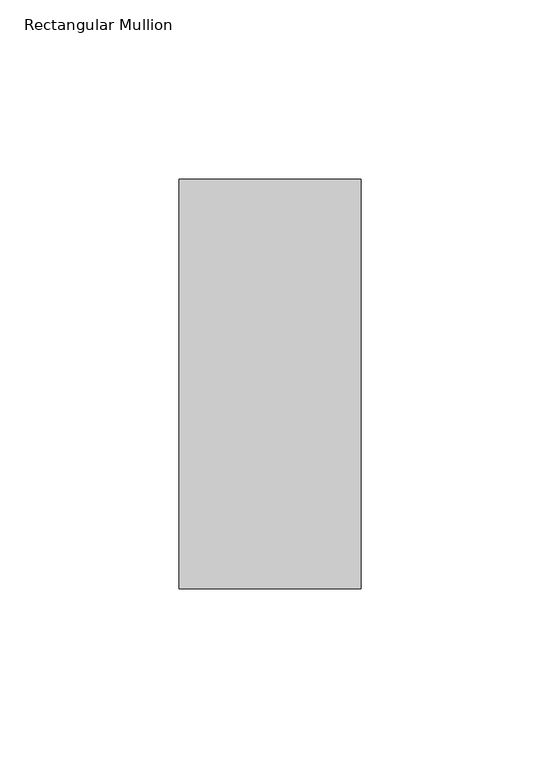
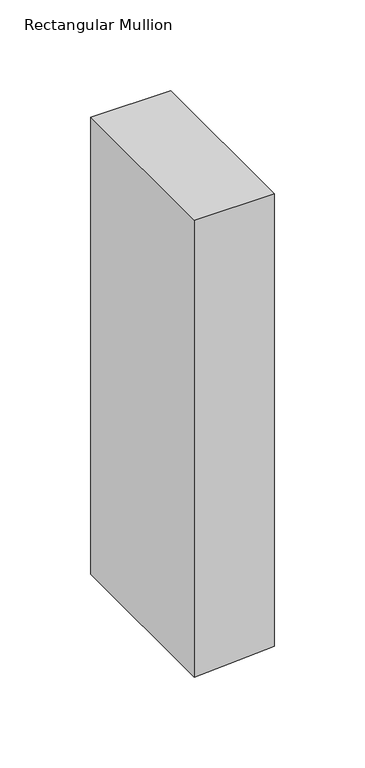
"""IFC4 building model written with IfcOpenShell, lengths in millimetres: member geometry, Rectangular Mullion : KAWNEER TRIFAB VERSAGLAZE 451T - CLEAR ANODIZED ALUM. - BACK GLAZED."""

from ifc_helpers import new_model, si_unit, frame, origin, place, context, project, spatial, polyline, outline, extrude, source, transform, mapped, element, save


def rectangular_mullion_3b3c7083(model_context):
    return source(origin(), model_context, "Body", "SweptSolid", [
        extrude(outline(polyline([(0.0, 25.4), (0.0, -25.4), (-307.5782217, -25.4), (-306.1887728, -3.1688169), (-304.4032217, 25.4), (0.0, 25.4)])), frame((0.0, -57.15, 0.0), z_axis=(0.0, 1.0, 0.0), x_axis=(0.0, 0.0, 1.0)), (0.0, 0.0, 1.0), 114.3),
    ])


if __name__ == "__main__":
    model = new_model("IFC4")
    model_context = context("Model", 3, world=origin())
    ifc_project = project(units=[si_unit("LENGTHUNIT", "METRE", prefix="MILLI")], contexts=[model_context])
    site = spatial("IfcSite", under=ifc_project)
    building = spatial("IfcBuilding", under=site)
    placement = place(None, origin())
    rectangular_mullion_shape = rectangular_mullion_3b3c7083(model_context)
    element("IfcMember", 1, ObjectType="Rectangular Mullion : KAWNEER TRIFAB VERSAGLAZE 451T - CLEAR ANODIZED ALUM. - BACK GLAZED", at=placement, inside=building, context=model_context, shape_type="MappedRepresentation", body=[
        mapped(rectangular_mullion_shape, transform((0.0, 0.0, 0.0), x_axis=(1.0, 0.0, 0.0), y_axis=(0.0, 1.0, 0.0), z_axis=(0.0, 0.0, 1.0))),
    ])
    save(model, "model.ifc")

# Revit data of these elements
# Type "Rectangular Mullion : KAWNEER TRIFAB VERSAGLAZE 451T - CLEAR ANODIZED ALUM. - BACK GLAZED"
#   built-in parameter 1007304 = 0.375 (stored number, unit not read)
#   built-in parameter 1007301 = 0.0833333 (stored number, unit not read)
#   built-in parameter 1007300 = 0.0833333 (stored number, unit not read)
# Element 1 (IfcMember, "Rectangular Mullion : KAWNEER TRIFAB VERSAGLAZE 451T - CLEAR ANODIZED ALUM. - BACK GLAZED")
#   Materials on its faces: "KAWNEER TRIFAB VERSAGLAZE 451T - CLEAR ANODIZED ALUM. - BACK GLAZED"
# Materials
#   "KAWNEER TRIFAB VERSAGLAZE 451T - CLEAR ANODIZED ALUM. - BACK GLAZED": class "Metal", colour RGB 244 244 244, transparency 0, Description = "Aluminum 6061", Cost = 0
